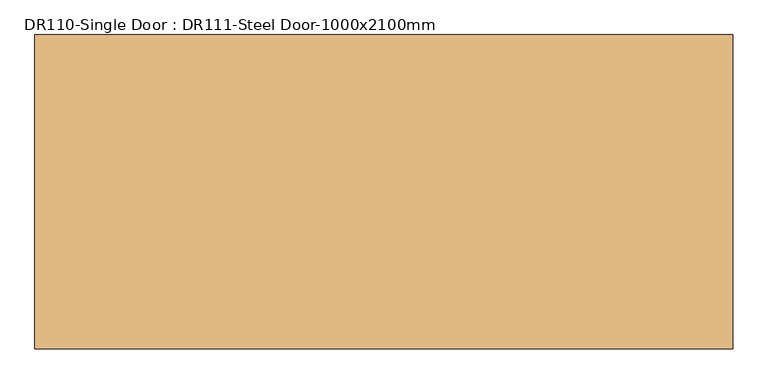
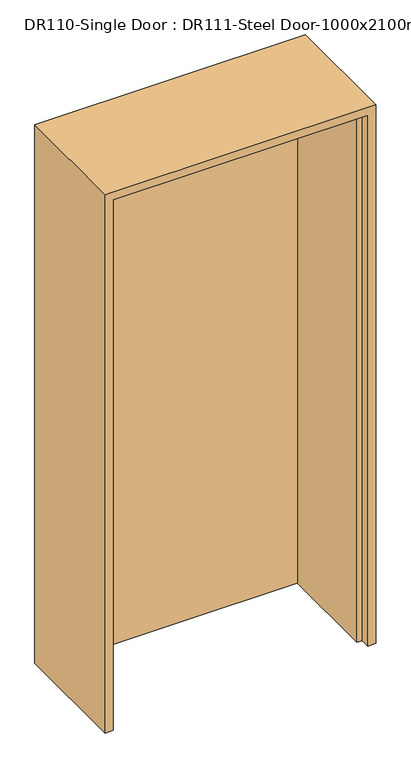
"""IFC4 building model written with IfcOpenShell, lengths in millimetres: door geometry, DR110-Single Door : DR111-Steel Door-1000x2100mm."""

import ifcopenshell
import ifcopenshell.guid

model = None  # the IFC model being written
_history = None  # IfcOwnerHistory: only IFC2X3 demands one
_inside = {}  # id of a spatial element -> (the spatial element, [elements in it])
_under = {}  # id of a project, library or spatial element -> (it, [spatial elements below it])
_declared = {}  # id of a project -> (the project, [libraries it declares])
_typed = {}  # id of a type object -> (the type object, [elements of that type])
_made_of = {}  # id of a material, layer set ... -> (it, [elements and type objects made of it])


def new_model(schema):
    """Start an empty IFC model of exactly this schema.

    Asked for "IFC4X3", IfcOpenShell would pick the latest addendum, in which some entities
    have other attributes; the version numbers below select the first issue.
    IFC2X3 requires an IfcOwnerHistory on every rooted entity: one is made here for all.
    """
    global model, _history
    if schema == "IFC4X3":
        model = ifcopenshell.file(schema_version=(4, 3, 0, 0))
    else:
        model = ifcopenshell.file(schema=schema)
    _inside.clear()
    _under.clear()
    _declared.clear()
    _typed.clear()
    _made_of.clear()
    _history = None
    if model.schema == "IFC2X3":
        org = make("IfcOrganization", Name="unknown")
        user = make(
            "IfcPersonAndOrganization",
            ThePerson=make("IfcPerson", FamilyName="unknown"),
            TheOrganization=org,
        )
        app = make(
            "IfcApplication",
            ApplicationDeveloper=org,
            Version="unknown",
            ApplicationFullName="unknown",
            ApplicationIdentifier="unknown",
        )
        _history = make(
            "IfcOwnerHistory",
            OwningUser=user,
            OwningApplication=app,
            ChangeAction="ADDED",
            CreationDate=0,
        )
    return model


def make(cls, **values):
    """One entity of the class cls with the attributes given. An attribute that is None is left unset."""
    return model.create_entity(
        cls, **{name: value for name, value in values.items() if value is not None}
    )


def rooted(cls, **values):
    """An entity with a GlobalId (a new one), such as an element, a storey or a relation."""
    return make(cls, GlobalId=ifcopenshell.guid.new(), OwnerHistory=_history, **values)


def si_unit(unit_type, name, prefix=None):
    """IfcSIUnit, for example si_unit("LENGTHUNIT", "METRE", prefix="MILLI")."""
    return make("IfcSIUnit", UnitType=unit_type, Prefix=prefix, Name=name)


def assignment(units):
    """IfcUnitAssignment: the units of a project."""
    return None if units is None else make("IfcUnitAssignment", Units=units)


def point(xyz):
    """IfcCartesianPoint."""
    return None if xyz is None else make("IfcCartesianPoint", Coordinates=xyz)


def direction(xyz):
    """IfcDirection."""
    return None if xyz is None else make("IfcDirection", DirectionRatios=xyz)


def frame(location, z_axis=None, x_axis=None):
    """IfcAxis2Placement3D, a coordinate frame: its origin and axes. An axis left out is left unset."""
    return make(
        "IfcAxis2Placement3D",
        Location=point(location),
        Axis=direction(z_axis),
        RefDirection=direction(x_axis),
    )


def origin():
    """The frame at (0, 0, 0) with its axes left unset."""
    return frame((0.0, 0.0, 0.0))


def origin_with_axes():
    """The frame at (0, 0, 0) with the z axis (0, 0, 1) and the x axis (1, 0, 0) written out."""
    return frame((0.0, 0.0, 0.0), z_axis=(0.0, 0.0, 1.0), x_axis=(1.0, 0.0, 0.0))


def place(relative_to, where):
    """IfcLocalPlacement: puts the frame where relative to a parent placement (None: the world)."""
    return make(
        "IfcLocalPlacement", PlacementRelTo=relative_to, RelativePlacement=where
    )


def context(
    kind, dimensions, precision=None, world=None, true_north=None, identifier=None
):
    """IfcGeometricRepresentationContext, for example the 3D "Model" context."""
    return make(
        "IfcGeometricRepresentationContext",
        ContextIdentifier=identifier,
        ContextType=kind,
        CoordinateSpaceDimension=dimensions,
        Precision=precision,
        WorldCoordinateSystem=world,
        TrueNorth=true_north,
    )


def project(units=None, contexts=None):
    """IfcProject with its units and contexts."""
    return rooted(
        "IfcProject",
        Name="project",
        RepresentationContexts=contexts,
        UnitsInContext=assignment(units),
    )


def spatial(cls, under=None, at=None, **own):
    """A site, building, storey or space (cls), placed at a placement, below another one or the project."""
    s = rooted(cls, ObjectPlacement=at, **own)
    if under is not None:
        _under.setdefault(under.id(), (under, []))[1].append(s)
    return s


def polyline(points):
    """IfcPolyline through the points."""
    return make("IfcPolyline", Points=[point(p) for p in points])


def outline(outer, holes=None, kind="AREA"):
    """IfcArbitraryClosedProfileDef: a profile drawn as a closed curve; with holes, ...WithVoids."""
    if holes is None:
        return make("IfcArbitraryClosedProfileDef", ProfileType=kind, OuterCurve=outer)
    return make(
        "IfcArbitraryProfileDefWithVoids",
        ProfileType=kind,
        OuterCurve=outer,
        InnerCurves=holes,
    )


def extrude(swept, where, along, depth):
    """IfcExtrudedAreaSolid: the profile swept, set in the frame where, extruded along a direction by depth."""
    return make(
        "IfcExtrudedAreaSolid",
        SweptArea=swept,
        Position=where,
        ExtrudedDirection=direction(along),
        Depth=depth,
    )


def faces_of(points, faces, orient=None, outer=None):
    """IfcFace entities. A face is a list of loops; a loop is a list of indices into points, from 0.

    orient and outer hold one flag for each loop. By default every Orientation is true, the
    first loop of a face is its IfcFaceOuterBound and the others are IfcFaceBound.
    """
    made = []
    for i, loops in enumerate(faces):
        bounds = []
        for j, loop in enumerate(loops):
            is_outer = j == 0 if outer is None else outer[i][j]
            bounds.append(
                make(
                    "IfcFaceOuterBound" if is_outer else "IfcFaceBound",
                    Bound=make("IfcPolyLoop", Polygon=[points[k] for k in loop]),
                    Orientation=True if orient is None else orient[i][j],
                )
            )
        made.append(make("IfcFace", Bounds=bounds))
    return made


def faceted_brep(points, faces, orient=None, outer=None, voids=None):
    """IfcFacetedBrep: a solid bounded by flat faces; with voids (closed shells), ...WithVoids."""
    shared = [point(p) for p in points]
    hull = make("IfcClosedShell", CfsFaces=faces_of(shared, faces, orient, outer))
    if voids is None:
        return make("IfcFacetedBrep", Outer=hull)
    return make(
        "IfcFacetedBrepWithVoids",
        Outer=hull,
        Voids=[
            make(cls, CfsFaces=faces_of(shared, fs, o, b)) for cls, fs, o, b in voids
        ],
    )


def shape(context_of_items, identifier, shape_type, items):
    """IfcShapeRepresentation: the items that make up one representation, for example the "Body"."""
    return make(
        "IfcShapeRepresentation",
        ContextOfItems=context_of_items,
        RepresentationIdentifier=identifier,
        RepresentationType=shape_type,
        Items=items,
    )


def source(mapping_origin, context_of_items, identifier, shape_type, items):
    """IfcRepresentationMap: a shape defined once, which mapped items show again and again."""
    return make(
        "IfcRepresentationMap",
        MappingOrigin=mapping_origin,
        MappedRepresentation=shape(context_of_items, identifier, shape_type, items),
    )


def transform(
    local_origin,
    x_axis=None,
    y_axis=None,
    z_axis=None,
    scale=None,
    scale2=None,
    scale3=None,
    uniform=True,
):
    """IfcCartesianTransformationOperator3D, or its non-uniform kind. x_axis, y_axis, z_axis: its Axis1, 2, 3."""
    if uniform:
        return make(
            "IfcCartesianTransformationOperator3D",
            Axis1=direction(x_axis),
            Axis2=direction(y_axis),
            LocalOrigin=point(local_origin),
            Scale=scale,
            Axis3=direction(z_axis),
        )
    return make(
        "IfcCartesianTransformationOperator3DnonUniform",
        Axis1=direction(x_axis),
        Axis2=direction(y_axis),
        LocalOrigin=point(local_origin),
        Scale=scale,
        Axis3=direction(z_axis),
        Scale2=scale2,
        Scale3=scale3,
    )


def mapped(mapping_source, mapping_target):
    """IfcMappedItem: shows the shape of a source again, moved by a transform."""
    return make(
        "IfcMappedItem", MappingSource=mapping_source, MappingTarget=mapping_target
    )


def made_of(thing, what):
    """Note that an element or type object is made of a material, layer set ...; save() writes the relation."""
    if what is not None:
        _made_of.setdefault(what.id(), (what, []))[1].append(thing)
    return thing


def element(
    cls,
    number,
    at=None,
    inside=None,
    cuts=None,
    type_object=None,
    material=None,
    context=None,
    identifier="Body",
    shape_type=None,
    held_by="IfcProductDefinitionShape",
    body=None,
    shapes=None,
    **own,
):
    """One element of the class cls, such as IfcWall. Its Tag is "e" and its number.

    at: its placement. inside: the storey or other place that contains it. cuts: it is an
    opening in that element (IfcRelVoidsElement). A single representation is given by context,
    identifier, shape_type and body (its items); several are given by shapes. held_by: the class
    of the entity that holds the representations. save() writes the other relations.
    """
    e = rooted(cls, Tag="e%d" % number, ObjectPlacement=at, **own)
    if body is not None:
        shapes = [shape(context, identifier, shape_type, body)]
    if shapes is not None:
        e.Representation = make(held_by, Representations=shapes)
    if inside is not None:
        _inside.setdefault(inside.id(), (inside, []))[1].append(e)
    if cuts is not None:
        rooted(
            "IfcRelVoidsElement", RelatingBuildingElement=cuts, RelatedOpeningElement=e
        )
    if type_object is not None:
        _typed.setdefault(type_object.id(), (type_object, []))[1].append(e)
    return made_of(e, material)


def aggregate(whole, parts):
    """IfcRelAggregates: a whole, such as a stair, and the parts it consists of."""
    return rooted("IfcRelAggregates", RelatingObject=whole, RelatedObjects=parts)


def save(model, path):
    """Write the relations noted so far, then the file.

    IfcRelAggregates (storeys below a building ...), IfcRelContainedInSpatialStructure (elements
    in a storey), IfcRelDefinesByType, IfcRelAssociatesMaterial and IfcRelDeclares: one each for
    every whole, place, type object, material and project.
    """
    for whole, parts in _under.values():
        aggregate(whole, parts)
    for where, things in _inside.values():
        rooted(
            "IfcRelContainedInSpatialStructure",
            RelatedElements=things,
            RelatingStructure=where,
        )
    for kind, things in _typed.values():
        rooted("IfcRelDefinesByType", RelatedObjects=things, RelatingType=kind)
    for what, things in _made_of.values():
        rooted("IfcRelAssociatesMaterial", RelatedObjects=things, RelatingMaterial=what)
    for by, libraries in _declared.values():
        rooted("IfcRelDeclares", RelatingContext=by, RelatedDefinitions=libraries)
    model.write(path)


def dr110_single_door_dr111_steel_door_1000x2100mm_e52ce95f(model_context):
    return source(origin(), model_context, "Body", "SolidModel", [
        extrude(outline(polyline([(470.0, 225.0), (470.0, 190.0), (-470.0, 190.0), (-470.0, 225.0), (470.0, 225.0)])), origin_with_axes(), (0.0, 0.0, 1.0), 2070.0),
        faceted_brep([(470.0, 225.0, 0.0), (500.0, 225.0, 0.0), (500.0, -225.0, 0.0), (470.0, -225.0, 0.0), (470.0, -190.0, 0.0), (450.0, -190.0, 0.0), (450.0, 190.0, 0.0), (470.0, 190.0, 0.0), (470.0, 225.0, 2070.0), (-470.0, 225.0, 2070.0), (-470.0, 225.0, 0.0), (-500.0, 225.0, 0.0), (-500.0, 225.0, 2100.0), (500.0, 225.0, 2100.0), (500.0, -225.0, 2100.0), (-500.0, -225.0, 2100.0), (-500.0, -225.0, 0.0), (-470.0, -225.0, 0.0), (-470.0, -225.0, 2070.0), (470.0, -225.0, 2070.0), (470.0, -190.0, 2070.0), (-470.0, -190.0, 2070.0), (-470.0, -190.0, 0.0), (-450.0, -190.0, 0.0), (-450.0, -190.0, 2050.0), (450.0, -190.0, 2050.0), (450.0, 190.0, 2050.0), (-450.0, 190.0, 2050.0), (-450.0, 190.0, 0.0), (-470.0, 190.0, 0.0), (-470.0, 190.0, 2070.0), (470.0, 190.0, 2070.0)], [[[0, 1, 2, 3, 4, 5, 6, 7]], [[1, 0, 8, 9, 10, 11, 12, 13]], [[2, 1, 13, 14]], [[3, 2, 14, 15, 16, 17, 18, 19]], [[4, 3, 19, 20]], [[5, 4, 20, 21, 22, 23, 24, 25]], [[6, 5, 25, 26]], [[7, 6, 26, 27, 28, 29, 30, 31]], [[0, 7, 31, 8]], [[9, 30, 29, 10]], [[10, 29, 28, 23, 22, 17, 16, 11]], [[15, 12, 11, 16]], [[21, 18, 17, 22]], [[27, 24, 23, 28]], [[14, 13, 12, 15]], [[20, 19, 18, 21]], [[26, 25, 24, 27]], [[8, 31, 30, 9]]]),
    ])


if __name__ == "__main__":
    model = new_model("IFC4")
    model_context = context("Model", 3, world=origin())
    ifc_project = project(units=[si_unit("LENGTHUNIT", "METRE", prefix="MILLI")], contexts=[model_context])
    site = spatial("IfcSite", under=ifc_project)
    building = spatial("IfcBuilding", under=site)
    placement = place(None, origin())
    dr110_single_door_dr111_steel_door_1000x2100mm_shape = dr110_single_door_dr111_steel_door_1000x2100mm_e52ce95f(model_context)
    element("IfcDoor", 1, ObjectType="DR110-Single Door : DR111-Steel Door-1000x2100mm", at=placement, inside=building, context=model_context, shape_type="MappedRepresentation", body=[
        mapped(dr110_single_door_dr111_steel_door_1000x2100mm_shape, transform((0.0, 0.0, 0.0), x_axis=(1.0, 0.0, 0.0), y_axis=(0.0, 1.0, 0.0), z_axis=(0.0, 0.0, 1.0))),
    ])
    save(model, "model.ifc")

# Revit data of these elements
# Type "DR110-Single Door : DR111-Steel Door-1000x2100mm"
#   Type Mark = "SD"
#   Analytic Construction = "<None>"
#   프레임 투영 외부. = 25 mm
#   프레임 투영 내부. = 25 mm
#   프레임 폭 = 75 mm
#   Height = 2100 mm
#   Width = 1000 mm
#   Define Thermal Properties by = 1
#   문 패널 = SD1 문 패널
#   문 프레임 = A04AQ098-00002_Steel Door_non FP_single
#   Function = (empty or 0)
#   Wall Closure = (empty or 0)
# Element 1 (IfcDoor, "DR110-Single Door : DR111-Steel Door-1000x2100mm")
#   Materials on its faces: "A04AQ098-00002_Steel Door_non FP_single", "SD1 문 패널"
# Materials
#   "SD1 문 패널": class "금속", colour RGB 247 247 247, transparency 0, Description = "STEEL DOOR (1000Wx2100H)"
#   "A04AQ098-00002_Steel Door_non FP_single": class "금속", colour RGB 247 247 247, transparency 0, Description = "Steel Door", W00) Work Master Code = "A04AQ098-00002", W01) Work Master_Lv1 = "Finishing Work", W02) Work Master_Lv2 = "Door & Window Work", W03) Work Master_Spec.1 = "Steel Door w/ Steel Frame", W04) Work Master_Spec.2 = "Fire Protective Rating: N/A, Single Door", W05) Work Master_Spec.3 = "w/ Hardware & Accessories", Cost = 0
